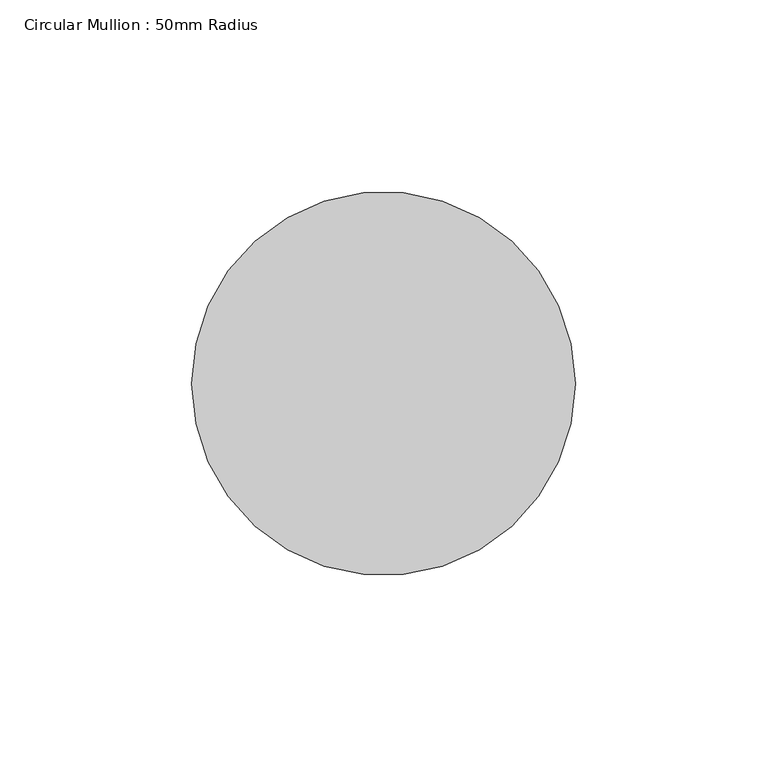
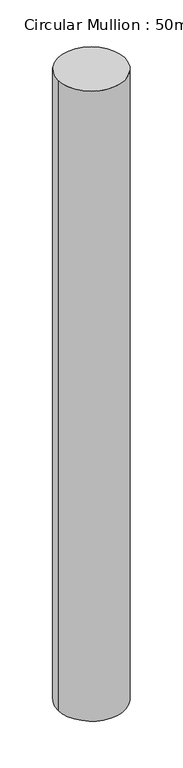
"""IFC4 building model written with IfcOpenShell, lengths in millimetres: member geometry, Circular Mullion : 50mm Radius."""

from ifc_helpers import new_model, si_unit, point, frame, origin, origin_2d, place, context, project, spatial, circle_curve, trimmed, segment, composite_curve, outline, extrude, source, transform, mapped, element, save


def circular_mullion_50mm_radius_23472ed7(model_context):
    return source(origin(), model_context, "Body", "SweptSolid", [
        extrude(outline(composite_curve([segment(trimmed(circle_curve(origin_2d(), 50.0), [point((50.0, 0.0))], [point((-50.0, 0.0))], False, "CARTESIAN"), True, "CONTINUOUS"), segment(trimmed(circle_curve(origin_2d(), 50.0), [point((-50.0, 0.0))], [point((50.0, 0.0))], False, "CARTESIAN"), True, "CONTINUOUS")], self_intersect=False)), frame((0.0, 0.0, -993.9810632), z_axis=(0.0, 0.0, 1.0), x_axis=(1.0, 0.0, 0.0)), (0.0, 0.0, 1.0), 993.9810632),
    ])


if __name__ == "__main__":
    model = new_model("IFC4")
    model_context = context("Model", 3, world=origin())
    ifc_project = project(units=[si_unit("LENGTHUNIT", "METRE", prefix="MILLI")], contexts=[model_context])
    site = spatial("IfcSite", under=ifc_project)
    building = spatial("IfcBuilding", under=site)
    placement = place(None, origin())
    circular_mullion_50mm_radius_shape = circular_mullion_50mm_radius_23472ed7(model_context)
    element("IfcMember", 1, ObjectType="Circular Mullion : 50mm Radius", at=placement, inside=building, context=model_context, shape_type="MappedRepresentation", body=[
        mapped(circular_mullion_50mm_radius_shape, transform((0.0, 0.0, 0.0), x_axis=(1.0, 0.0, 0.0), y_axis=(0.0, 1.0, 0.0), z_axis=(0.0, 0.0, 1.0))),
    ])
    save(model, "model.ifc")

# Revit data of these elements
# Type "Circular Mullion : 50mm Radius"
#   built-in parameter 1007350 = 0.164042 (stored number, unit not read)
# Element 1 (IfcMember, "Circular Mullion : 50mm Radius")
#   Materials on its faces: "Aluminium"
# Materials
#   "Aluminium": class "Metal", colour RGB 247 247 247, transparency 0, Description = "Aluminium 6061", Cost = 0
